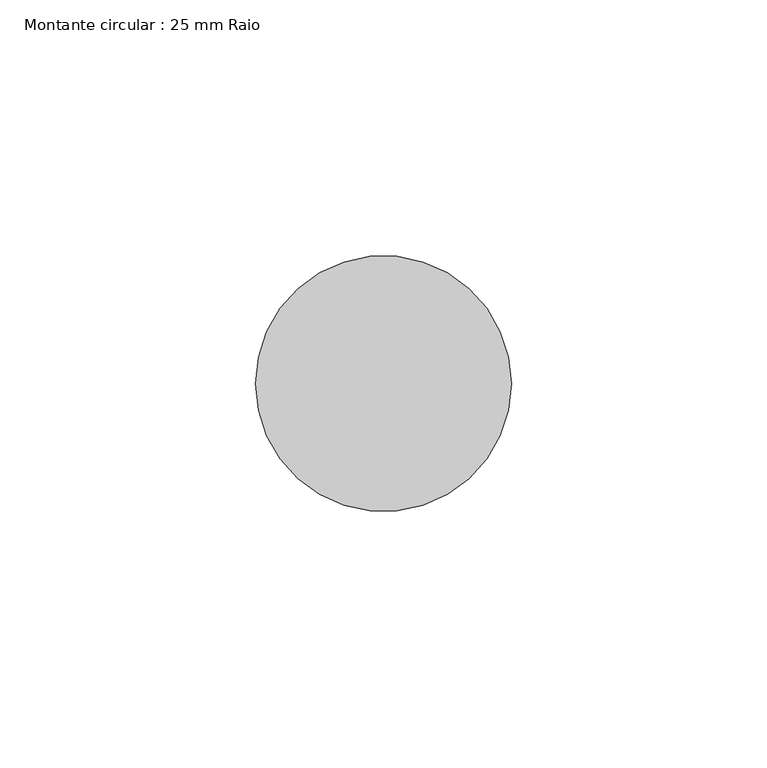
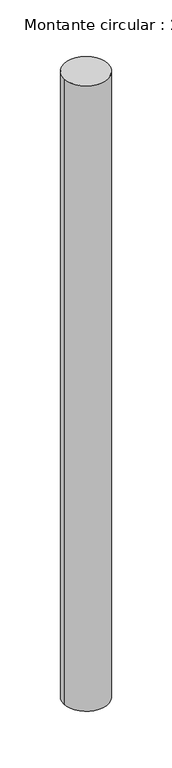
"""IFC4 building model written with IfcOpenShell, lengths in millimetres: member geometry, Montante circular : 25 mm Raio."""

from ifc_helpers import new_model, si_unit, point, frame, origin, origin_2d, place, context, project, spatial, circle_curve, trimmed, segment, composite_curve, outline, extrude, source, transform, mapped, element, save


def montante_circular_25_mm_raio_7488278f(model_context):
    return source(origin(), model_context, "Body", "SweptSolid", [
        extrude(outline(composite_curve([segment(trimmed(circle_curve(origin_2d(), 25.0), [point((25.0, 0.0))], [point((-25.0, 0.0))], False, "CARTESIAN"), True, "CONTINUOUS"), segment(trimmed(circle_curve(origin_2d(), 25.0), [point((-25.0, 0.0))], [point((25.0, 0.0))], False, "CARTESIAN"), True, "CONTINUOUS")], self_intersect=False)), frame((0.0, 0.0, -745.3587969), z_axis=(0.0, 0.0, 1.0), x_axis=(1.0, 0.0, 0.0)), (0.0, 0.0, 1.0), 745.3587969),
    ])


if __name__ == "__main__":
    model = new_model("IFC4")
    model_context = context("Model", 3, world=origin())
    ifc_project = project(units=[si_unit("LENGTHUNIT", "METRE", prefix="MILLI")], contexts=[model_context])
    site = spatial("IfcSite", under=ifc_project)
    building = spatial("IfcBuilding", under=site)
    placement = place(None, origin())
    montante_circular_25_mm_raio_shape = montante_circular_25_mm_raio_7488278f(model_context)
    element("IfcMember", 1, ObjectType="Montante circular : 25 mm Raio", at=placement, inside=building, context=model_context, shape_type="MappedRepresentation", body=[
        mapped(montante_circular_25_mm_raio_shape, transform((0.0, 0.0, 0.0), x_axis=(1.0, 0.0, 0.0), y_axis=(0.0, 1.0, 0.0), z_axis=(0.0, 0.0, 1.0))),
    ])
    save(model, "model.ifc")

# Revit data of these elements
# Type "Montante circular : 25 mm Raio"
#   built-in parameter 1007350 = 0.082021 (stored number, unit not read)
# Element 1 (IfcMember, "Montante circular : 25 mm Raio")
#   Materials on its faces: "Alumín."
# Materials
#   "Alumín.": class "Metal", colour RGB 247 247 247, transparency 0, Description = "Alumín. 6061", Cost = 0
